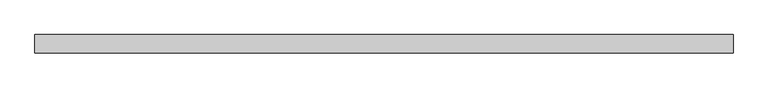
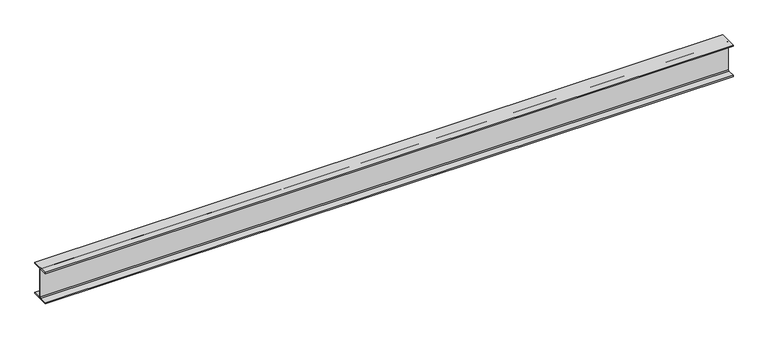
"""IFC4 building model written with IfcOpenShell, lengths in millimetres: beam geometry, Old_Steel Beam_H-KSD3502 : H_SB_ASB_H-482×300x11x15."""

from ifc_helpers import new_model, si_unit, point, frame, frame_2d, origin, place, context, project, spatial, polyline, circle_curve, trimmed, segment, composite_curve, outline, extrude, source, transform, mapped, element, save


def beam_c818b0c6(model_context):
    return source(origin(), model_context, "Body", "SweptSolid", [
        extrude(outline(composite_curve([segment(polyline([(82.5, -141.5), (82.5, -151.7), (-82.5, -151.7), (-82.5, -141.5), (-11.9, -141.5)]), True, "CONTINUOUS"), segment(trimmed(circle_curve(frame_2d((-11.9, -132.6)), 8.9), [point((-11.9, -141.5))], [point((-3.0, -132.6))], True, "CARTESIAN"), True, "CONTINUOUS"), segment(polyline([(-3.0, -132.6), (-3.0, 132.6)]), True, "CONTINUOUS"), segment(trimmed(circle_curve(frame_2d((-11.9, 132.6)), 8.9), [point((-3.0, 132.6))], [point((-11.9, 141.5))], True, "CARTESIAN"), True, "CONTINUOUS"), segment(polyline([(-11.9, 141.5), (-82.5, 141.5), (-82.5, 151.7), (82.5, 151.7), (82.5, 141.5), (11.9, 141.5)]), True, "CONTINUOUS"), segment(trimmed(circle_curve(frame_2d((11.9, 132.6)), 8.9), [point((11.9, 141.5))], [point((3.0, 132.6))], True, "CARTESIAN"), True, "CONTINUOUS"), segment(polyline([(3.0, 132.6), (3.0, -132.6)]), True, "CONTINUOUS"), segment(trimmed(circle_curve(frame_2d((11.9, -132.6)), 8.9), [point((3.0, -132.6))], [point((11.9, -141.5))], True, "CARTESIAN"), True, "CONTINUOUS"), segment(polyline([(11.9, -141.5), (82.5, -141.5)]), True, "CONTINUOUS")], self_intersect=False)), frame((-3154.8, 0.0, 0.0), z_axis=(1.0, 0.0, 0.0), x_axis=(0.0, 1.0, 0.0)), (0.0, 0.0, 1.0), 6309.6),
    ])


if __name__ == "__main__":
    model = new_model("IFC4")
    model_context = context("Model", 3, world=origin())
    ifc_project = project(units=[si_unit("LENGTHUNIT", "METRE", prefix="MILLI")], contexts=[model_context])
    site = spatial("IfcSite", under=ifc_project)
    building = spatial("IfcBuilding", under=site)
    placement = place(None, origin())
    beam_shape = beam_c818b0c6(model_context)
    element("IfcBeam", 1, ObjectType="Old_Steel Beam_H-KSD3502 : H_SB_ASB_H-482×300x11x15", at=placement, inside=building, context=model_context, shape_type="MappedRepresentation", body=[
        mapped(beam_shape, transform((0.0, 0.0, 0.0), x_axis=(1.0, 0.0, 0.0), y_axis=(0.0, 1.0, 0.0), z_axis=(0.0, 0.0, 1.0))),
    ])
    save(model, "model.ifc")

# Revit data of these elements
# Type "Old_Steel Beam_H-KSD3502 : H_SB_ASB_H-482×300x11x15"
#   Width = 30.0 cm
#   Web Thickness = 1.1 cm
#   Web Fillet = 2.6 cm
#   Warping Constant = 3680250.0 cm⁶
#   Torsional Moment of Inertia = 88.2192 cm⁴
#   Torsional Modulus = 1.0 cm³
#   Section Area = 145.5 cm²
#   Plastic Modulus weak axis = 695.0 cm³
#   Plastic Modulus strong axis = 2790.0 cm³
#   Perimeter = 2.10 m²/m
#   Nominal Weight = 114.00 kgf/m
#   Moment of Inertia weak axis = 6760.00 cm⁴
#   Moment of Inertia strong axis = 60400.00 cm⁴
#   Height = 48.2 cm
#   Flange Thickness = 1.5 cm
#   Elastic Modulus weak axis = 451.0 cm³
#   Elastic Modulus strong axis = 2500.0 cm³
#   Centroid Vertical = 24.1 cm
#   Centroid Horizontal = 15.0 cm
#   Length [instance default] = 1.5240 m
#   Structural Material [instance default] = Steel, 45-345
#   Assembly Code = ""
# Element 1 (IfcBeam, "Old_Steel Beam_H-KSD3502 : H_SB_ASB_H-482×300x11x15")
#   Structural Material = none
# Materials
#   "Steel, 45-345": class "Metal", colour RGB 189 187 185, transparency 0, Description = "Steel 345 MPa", Cost = 0
